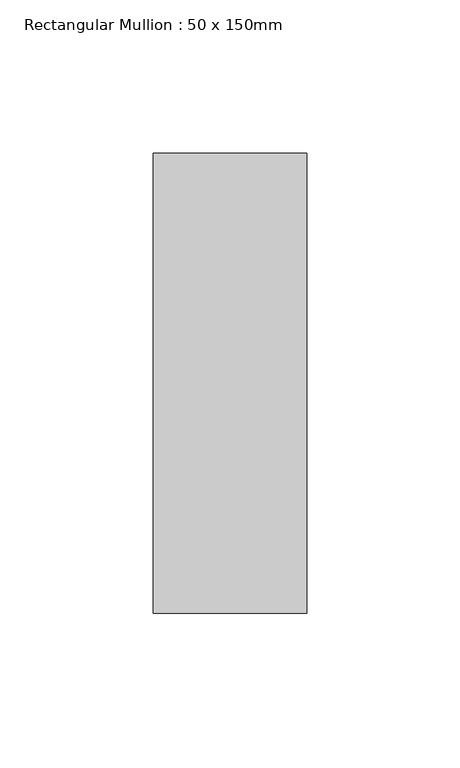
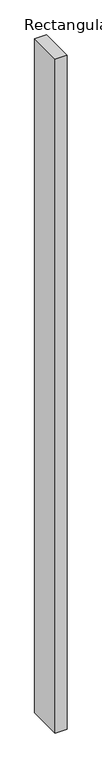
"""IFC4 building model written with IfcOpenShell, lengths in millimetres: member geometry, Rectangular Mullion : 50 x 150mm."""

from ifc_helpers import new_model, si_unit, frame, origin, place, context, project, spatial, polyline, outline, extrude, source, transform, mapped, element, save


def rectangular_mullion_50_x_150mm_6c7cb899(model_context):
    return source(origin(), model_context, "Body", "SweptSolid", [
        extrude(outline(polyline([(25.0, 75.0), (25.0, -75.0), (-25.0, -75.0), (-25.0, 75.0), (25.0, 75.0)])), frame((0.0, 0.0, -3000.0), z_axis=(0.0, 0.0, 1.0), x_axis=(1.0, 0.0, 0.0)), (0.0, 0.0, 1.0), 3000.0),
    ])


if __name__ == "__main__":
    model = new_model("IFC4")
    model_context = context("Model", 3, world=origin())
    ifc_project = project(units=[si_unit("LENGTHUNIT", "METRE", prefix="MILLI")], contexts=[model_context])
    site = spatial("IfcSite", under=ifc_project)
    building = spatial("IfcBuilding", under=site)
    placement = place(None, origin())
    rectangular_mullion_50_x_150mm_shape = rectangular_mullion_50_x_150mm_6c7cb899(model_context)
    element("IfcMember", 1, ObjectType="Rectangular Mullion : 50 x 150mm", at=placement, inside=building, context=model_context, shape_type="MappedRepresentation", body=[
        mapped(rectangular_mullion_50_x_150mm_shape, transform((0.0, 0.0, 0.0), x_axis=(1.0, 0.0, 0.0), y_axis=(0.0, 1.0, 0.0), z_axis=(0.0, 0.0, 1.0))),
    ])
    save(model, "model.ifc")

# Revit data of these elements
# Type "Rectangular Mullion : 50 x 150mm"
#   built-in parameter 1007304 = 0.492126 (stored number, unit not read)
#   built-in parameter 1007301 = 0.082021 (stored number, unit not read)
#   built-in parameter 1007300 = 0.082021 (stored number, unit not read)
# Element 1 (IfcMember, "Rectangular Mullion : 50 x 150mm")
#   Materials on its faces: "Metal - Aluminium"
# Materials
#   "Metal - Aluminium": class "Metal", colour RGB 247 247 247, transparency 0
